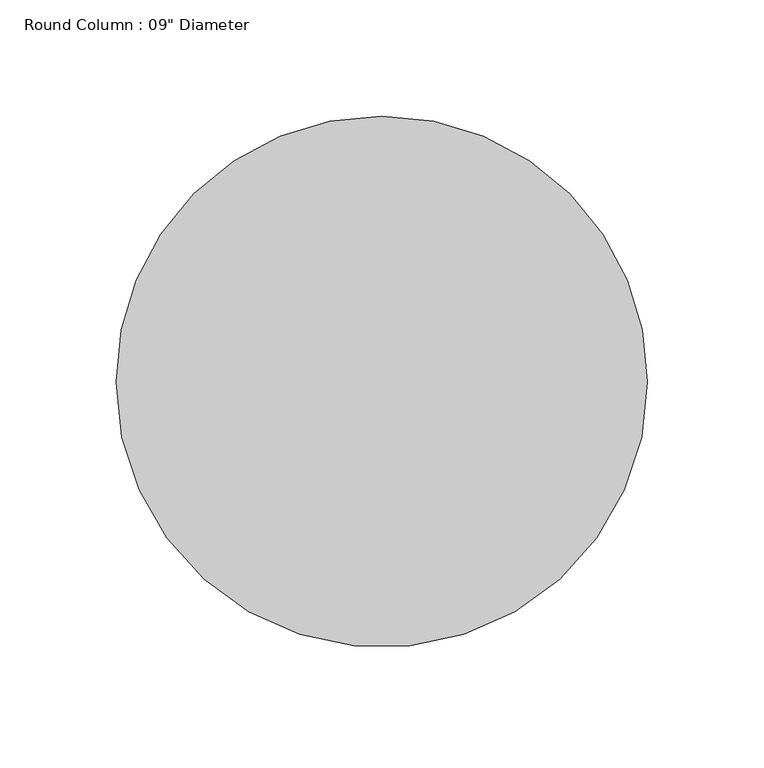
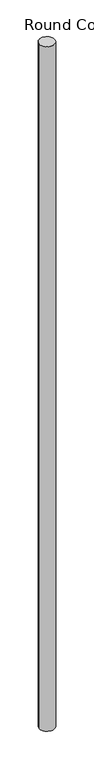
"""IFC4 building model written with IfcOpenShell, lengths in millimetres: column geometry."""

from ifc_helpers import new_model, si_unit, point, frame, origin, origin_2d, place, context, project, spatial, circle_curve, trimmed, segment, composite_curve, outline, extrude, source, transform, mapped, element, save


def column_b076e593(model_context):
    return source(origin(), model_context, "Body", "SweptSolid", [
        extrude(outline(composite_curve([segment(trimmed(circle_curve(origin_2d(), 114.3), [point((114.3, 0.0))], [point((-114.3, 0.0))], False, "CARTESIAN"), True, "CONTINUOUS"), segment(trimmed(circle_curve(origin_2d(), 114.3), [point((-114.3, 0.0))], [point((0.0, 114.3))], False, "CARTESIAN"), True, "CONTINUOUS"), segment(trimmed(circle_curve(origin_2d(), 114.3), [point((0.0, 114.3))], [point((114.3, 0.0))], False, "CARTESIAN"), True, "CONTINUOUS")], self_intersect=False)), frame((0.0, 0.0, 30327.6), z_axis=(0.0, 0.0, 1.0), x_axis=(1.0, 0.0, 0.0)), (0.0, 0.0, 1.0), 10922.0),
    ])


if __name__ == "__main__":
    model = new_model("IFC4")
    model_context = context("Model", 3, world=origin())
    ifc_project = project(units=[si_unit("LENGTHUNIT", "METRE", prefix="MILLI")], contexts=[model_context])
    site = spatial("IfcSite", under=ifc_project)
    building = spatial("IfcBuilding", under=site)
    placement = place(None, origin())
    column_shape = column_b076e593(model_context)
    element("IfcColumn", 1, ObjectType="Round Column : 09\" Diameter", at=placement, inside=building, context=model_context, shape_type="MappedRepresentation", body=[
        mapped(column_shape, transform((0.0, 0.0, 0.0), x_axis=(1.0, 0.0, 0.0), y_axis=(0.0, 1.0, 0.0), z_axis=(0.0, 0.0, 1.0))),
    ])
    save(model, "model.ifc")

# Revit data of these elements
# Type "Round Column : 09\" Diameter"
#   Assembly Code = "B1010200"
#   Diameter = 0' - 9"
#   Offset Base = 0' - 0"
#   Offset Top = 0' - 0"
#   Material = Metal - Aluminum
# Element 1 (IfcColumn, "Round Column : 09\" Diameter")
#   Materials on its faces: "Metal - Aluminum"
# Materials
#   "Metal - Aluminum": class "Metal", colour RGB 109 108 108, transparency 0
